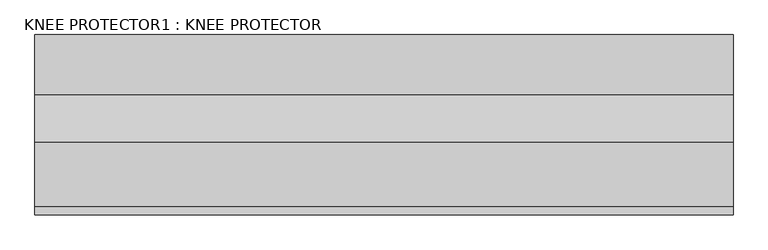
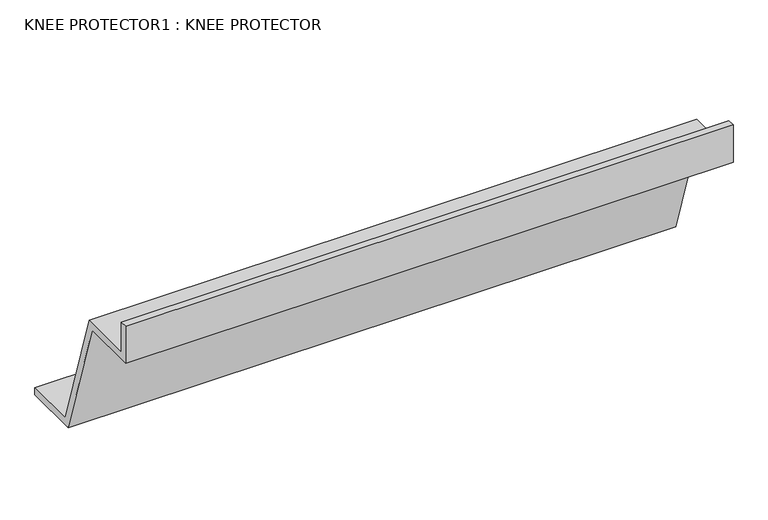
"""IFC4 building model written with IfcOpenShell, lengths in millimetres: furniture geometry, KNEE PROTECTOR1 : KNEE PROTECTOR."""

from ifc_helpers import new_model, si_unit, frame, origin, place, context, project, spatial, polyline, outline, extrude, source, transform, mapped, element, save


def knee_protector1_knee_protector_1c145a6a(model_context):
    return source(origin(), model_context, "Body", "SweptSolid", [
        extrude(outline(polyline([(-237028.2315414, 685.8), (-237028.2315414, 825.5), (-237002.8315414, 825.5), (-237002.8315414, 711.2), (-236803.9902606, 711.2), (-236655.4369755, 254.0), (-236469.4315414, 254.0), (-236469.4315414, 228.6), (-236673.8911557, 228.6), (-236822.4444408, 685.8), (-237028.2315414, 685.8)])), frame((610620.0458295, 0.0, 0.0), z_axis=(1.0, 0.0, 0.0), x_axis=(0.0, 1.0, 0.0)), (0.0, 0.0, 1.0), 2162.175),
    ])


if __name__ == "__main__":
    model = new_model("IFC4")
    model_context = context("Model", 3, world=origin())
    ifc_project = project(units=[si_unit("LENGTHUNIT", "METRE", prefix="MILLI")], contexts=[model_context])
    site = spatial("IfcSite", under=ifc_project)
    building = spatial("IfcBuilding", under=site)
    placement = place(None, origin())
    knee_protector1_knee_protector_shape = knee_protector1_knee_protector_1c145a6a(model_context)
    element("IfcFurniture", 1, ObjectType="KNEE PROTECTOR1 : KNEE PROTECTOR", at=placement, inside=building, context=model_context, shape_type="MappedRepresentation", body=[
        mapped(knee_protector1_knee_protector_shape, transform((0.0, 0.0, 0.0), x_axis=(1.0, 0.0, 0.0), y_axis=(0.0, 1.0, 0.0), z_axis=(0.0, 0.0, 1.0))),
    ])
    save(model, "model.ifc")

# Revit data of these elements
# Element 1 (IfcFurniture, "KNEE PROTECTOR1 : KNEE PROTECTOR")
#   Materials on its faces: "CASEWORK"
# Materials
#   "CASEWORK": class "Generic", colour RGB 181 181 181, transparency 0, Cost = 0
